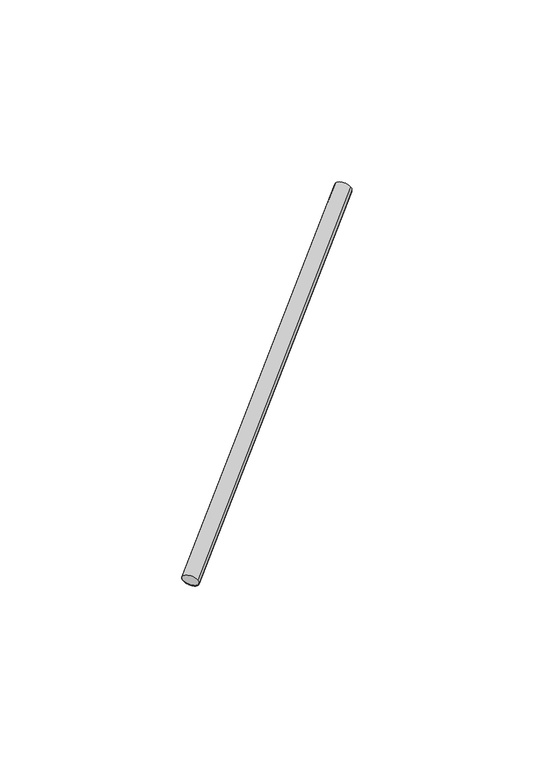
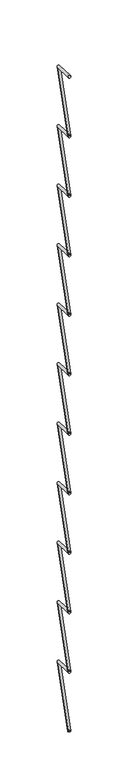
"""IFC4 building model written with IfcOpenShell, lengths in millimetres: proxy geometry, Vigota 7 (Pano 3) (Mf = 137)."""

from ifc_helpers import new_model, si_unit, point, frame, origin, origin_2d, place, context, project, spatial, circle_curve, trimmed, segment, composite_curve, outline, extrude, source, transform, mapped, element, save


def structural_framing_98597a9d(model_context):
    return source(origin(), model_context, "Body", "SweptSolid", [
        extrude(outline(composite_curve([segment(trimmed(circle_curve(origin_2d(), 2.5), [point((2.5, 0.0))], [point((-2.5, 0.0))], False, "CARTESIAN"), True, "CONTINUOUS"), segment(trimmed(circle_curve(origin_2d(), 2.5), [point((-2.5, 0.0))], [point((2.5, 0.0))], False, "CARTESIAN"), True, "CONTINUOUS")], self_intersect=False)), frame((-42.0, 0.0, 1737.500535), z_axis=(0.3218603428886276, 0.8276408817707567, 0.4598004898837537), x_axis=(0.8192319205108605, 3.936835275445103e-11, -0.5734623443750141)), (0.0, 0.0, 1.0), 130.491379),
        extrude(outline(composite_curve([segment(trimmed(circle_curve(origin_2d(), 2.5), [point((2.5, 0.0))], [point((-2.5, 0.0))], False, "CARTESIAN"), True, "CONTINUOUS"), segment(trimmed(circle_curve(origin_2d(), 2.5), [point((-2.5, 0.0))], [point((2.5, 0.0))], False, "CARTESIAN"), True, "CONTINUOUS")], self_intersect=False)), frame((0.0, 108.0, 1797.500535), z_axis=(-0.3218603428886276, -0.8276408817707567, 0.4598004898837537), x_axis=(0.8192319205108605, 3.936835275445103e-11, 0.5734623443750141)), (0.0, 0.0, 1.0), 130.491379),
        extrude(outline(composite_curve([segment(trimmed(circle_curve(origin_2d(), 2.5), [point((2.5, 0.0))], [point((-2.5, 0.0))], False, "CARTESIAN"), True, "CONTINUOUS"), segment(trimmed(circle_curve(origin_2d(), 2.5), [point((-2.5, 0.0))], [point((2.5, 0.0))], False, "CARTESIAN"), True, "CONTINUOUS")], self_intersect=False)), frame((-42.0, 0.0, 1857.500535), z_axis=(0.3218603428886276, 0.8276408817707567, 0.4598004898837537), x_axis=(0.8192319205108605, 3.936835275445103e-11, -0.5734623443750141)), (0.0, 0.0, 1.0), 130.491379),
        extrude(outline(composite_curve([segment(trimmed(circle_curve(origin_2d(), 2.5), [point((2.5, 0.0))], [point((-2.5, 0.0))], False, "CARTESIAN"), True, "CONTINUOUS"), segment(trimmed(circle_curve(origin_2d(), 2.5), [point((-2.5, 0.0))], [point((2.5, 0.0))], False, "CARTESIAN"), True, "CONTINUOUS")], self_intersect=False)), frame((0.0, 108.0, 1917.500535), z_axis=(-0.3218603428886276, -0.8276408817707567, 0.4598004898837537), x_axis=(0.8192319205108605, 3.936835275445103e-11, 0.5734623443750141)), (0.0, 0.0, 1.0), 130.491379),
        extrude(outline(composite_curve([segment(trimmed(circle_curve(origin_2d(), 2.5), [point((2.5, 0.0))], [point((-2.5, 0.0))], False, "CARTESIAN"), True, "CONTINUOUS"), segment(trimmed(circle_curve(origin_2d(), 2.5), [point((-2.5, 0.0))], [point((2.5, 0.0))], False, "CARTESIAN"), True, "CONTINUOUS")], self_intersect=False)), frame((-42.0, 0.0, 1977.500535), z_axis=(0.3218603428886276, 0.8276408817707567, 0.4598004898837537), x_axis=(0.8192319205108605, 3.936835275445103e-11, -0.5734623443750141)), (0.0, 0.0, 1.0), 130.491379),
        extrude(outline(composite_curve([segment(trimmed(circle_curve(origin_2d(), 2.5), [point((2.5, 0.0))], [point((-2.5, 0.0))], False, "CARTESIAN"), True, "CONTINUOUS"), segment(trimmed(circle_curve(origin_2d(), 2.5), [point((-2.5, 0.0))], [point((2.5, 0.0))], False, "CARTESIAN"), True, "CONTINUOUS")], self_intersect=False)), frame((0.0, 108.0, 2037.500535), z_axis=(-0.3218603428886276, -0.8276408817707567, 0.4598004898837537), x_axis=(0.8192319205108605, 3.936835275445103e-11, 0.5734623443750141)), (0.0, 0.0, 1.0), 130.491379),
        extrude(outline(composite_curve([segment(trimmed(circle_curve(origin_2d(), 2.5), [point((2.5, 0.0))], [point((-2.5, 0.0))], False, "CARTESIAN"), True, "CONTINUOUS"), segment(trimmed(circle_curve(origin_2d(), 2.5), [point((-2.5, 0.0))], [point((2.5, 0.0))], False, "CARTESIAN"), True, "CONTINUOUS")], self_intersect=False)), frame((-42.0, 0.0, 2097.500535), z_axis=(0.3218603428886276, 0.8276408817707567, 0.4598004898837537), x_axis=(0.8192319205108605, 3.936835275445103e-11, -0.5734623443750141)), (0.0, 0.0, 1.0), 130.491379),
        extrude(outline(composite_curve([segment(trimmed(circle_curve(origin_2d(), 2.5), [point((2.5, 0.0))], [point((-2.5, 0.0))], False, "CARTESIAN"), True, "CONTINUOUS"), segment(trimmed(circle_curve(origin_2d(), 2.5), [point((-2.5, 0.0))], [point((2.5, 0.0))], False, "CARTESIAN"), True, "CONTINUOUS")], self_intersect=False)), frame((0.0, 108.0, 2157.500535), z_axis=(-0.3218603428886276, -0.8276408817707567, 0.4598004898837537), x_axis=(0.8192319205108605, 3.936835275445103e-11, 0.5734623443750141)), (0.0, 0.0, 1.0), 130.491379),
        extrude(outline(composite_curve([segment(trimmed(circle_curve(origin_2d(), 2.5), [point((2.5, 0.0))], [point((-2.5, 0.0))], False, "CARTESIAN"), True, "CONTINUOUS"), segment(trimmed(circle_curve(origin_2d(), 2.5), [point((-2.5, 0.0))], [point((2.5, 0.0))], False, "CARTESIAN"), True, "CONTINUOUS")], self_intersect=False)), frame((-42.0, 0.0, 2217.500535), z_axis=(0.3218603428886276, 0.8276408817707567, 0.4598004898837537), x_axis=(0.8192319205108605, 3.936835275445103e-11, -0.5734623443750141)), (0.0, 0.0, 1.0), 130.491379),
        extrude(outline(composite_curve([segment(trimmed(circle_curve(origin_2d(), 2.5), [point((2.5, 0.0))], [point((-2.5, 0.0))], False, "CARTESIAN"), True, "CONTINUOUS"), segment(trimmed(circle_curve(origin_2d(), 2.5), [point((-2.5, 0.0))], [point((2.5, 0.0))], False, "CARTESIAN"), True, "CONTINUOUS")], self_intersect=False)), frame((0.0, 108.0, 2277.500535), z_axis=(-0.3218603428886276, -0.8276408817707567, 0.4598004898837537), x_axis=(0.8192319205108605, 3.936835275445103e-11, 0.5734623443750141)), (0.0, 0.0, 1.0), 130.491379),
        extrude(outline(composite_curve([segment(trimmed(circle_curve(origin_2d(), 2.5), [point((2.5, 0.0))], [point((-2.5, 0.0))], False, "CARTESIAN"), True, "CONTINUOUS"), segment(trimmed(circle_curve(origin_2d(), 2.5), [point((-2.5, 0.0))], [point((2.5, 0.0))], False, "CARTESIAN"), True, "CONTINUOUS")], self_intersect=False)), frame((-42.0, 0.0, 2337.500535), z_axis=(0.3218603428886276, 0.8276408817707567, 0.4598004898837537), x_axis=(0.8192319205108605, 3.936835275445103e-11, -0.5734623443750141)), (0.0, 0.0, 1.0), 130.491379),
        extrude(outline(composite_curve([segment(trimmed(circle_curve(origin_2d(), 2.5), [point((2.5, 0.0))], [point((-2.5, 0.0))], False, "CARTESIAN"), True, "CONTINUOUS"), segment(trimmed(circle_curve(origin_2d(), 2.5), [point((-2.5, 0.0))], [point((2.5, 0.0))], False, "CARTESIAN"), True, "CONTINUOUS")], self_intersect=False)), frame((0.0, 108.0, 2397.500535), z_axis=(-0.3218603428886276, -0.8276408817707567, 0.4598004898837537), x_axis=(0.8192319205108605, 3.936835275445103e-11, 0.5734623443750141)), (0.0, 0.0, 1.0), 130.491379),
        extrude(outline(composite_curve([segment(trimmed(circle_curve(origin_2d(), 2.5), [point((2.5, 0.0))], [point((-2.5, 0.0))], False, "CARTESIAN"), True, "CONTINUOUS"), segment(trimmed(circle_curve(origin_2d(), 2.5), [point((-2.5, 0.0))], [point((2.5, 0.0))], False, "CARTESIAN"), True, "CONTINUOUS")], self_intersect=False)), frame((-42.0, 0.0, 2457.500535), z_axis=(0.3218603428886276, 0.8276408817707567, 0.4598004898837537), x_axis=(0.8192319205108605, 3.936835275445103e-11, -0.5734623443750141)), (0.0, 0.0, 1.0), 130.491379),
        extrude(outline(composite_curve([segment(trimmed(circle_curve(origin_2d(), 2.5), [point((2.5, 0.0))], [point((-2.5, 0.0))], False, "CARTESIAN"), True, "CONTINUOUS"), segment(trimmed(circle_curve(origin_2d(), 2.5), [point((-2.5, 0.0))], [point((2.5, 0.0))], False, "CARTESIAN"), True, "CONTINUOUS")], self_intersect=False)), frame((0.0, 108.0, 2517.500535), z_axis=(-0.3218603428886276, -0.8276408817707567, 0.4598004898837537), x_axis=(0.8192319205108605, 3.936835275445103e-11, 0.5734623443750141)), (0.0, 0.0, 1.0), 130.491379),
        extrude(outline(composite_curve([segment(trimmed(circle_curve(origin_2d(), 2.5), [point((2.5, 0.0))], [point((-2.5, 0.0))], False, "CARTESIAN"), True, "CONTINUOUS"), segment(trimmed(circle_curve(origin_2d(), 2.5), [point((-2.5, 0.0))], [point((2.5, 0.0))], False, "CARTESIAN"), True, "CONTINUOUS")], self_intersect=False)), frame((-42.0, 0.0, 2577.500535), z_axis=(0.3218603428886276, 0.8276408817707567, 0.4598004898837537), x_axis=(0.8192319205108605, 3.936835275445103e-11, -0.5734623443750141)), (0.0, 0.0, 1.0), 130.491379),
        extrude(outline(composite_curve([segment(trimmed(circle_curve(origin_2d(), 2.5), [point((2.5, 0.0))], [point((-2.5, 0.0))], False, "CARTESIAN"), True, "CONTINUOUS"), segment(trimmed(circle_curve(origin_2d(), 2.5), [point((-2.5, 0.0))], [point((2.5, 0.0))], False, "CARTESIAN"), True, "CONTINUOUS")], self_intersect=False)), frame((0.0, 108.0, 2637.500535), z_axis=(-0.3218603428886276, -0.8276408817707567, 0.4598004898837537), x_axis=(0.8192319205108605, 3.936835275445103e-11, 0.5734623443750141)), (0.0, 0.0, 1.0), 130.491379),
        extrude(outline(composite_curve([segment(trimmed(circle_curve(origin_2d(), 2.5), [point((2.5, 0.0))], [point((-2.5, 0.0))], False, "CARTESIAN"), True, "CONTINUOUS"), segment(trimmed(circle_curve(origin_2d(), 2.5), [point((-2.5, 0.0))], [point((2.5, 0.0))], False, "CARTESIAN"), True, "CONTINUOUS")], self_intersect=False)), frame((-42.0, 0.0, 2697.500535), z_axis=(0.3218603428886276, 0.8276408817707567, 0.4598004898837537), x_axis=(0.8192319205108605, 3.936835275445103e-11, -0.5734623443750141)), (0.0, 0.0, 1.0), 130.491379),
        extrude(outline(composite_curve([segment(trimmed(circle_curve(origin_2d(), 2.5), [point((2.5, 0.0))], [point((-2.5, 0.0))], False, "CARTESIAN"), True, "CONTINUOUS"), segment(trimmed(circle_curve(origin_2d(), 2.5), [point((-2.5, 0.0))], [point((2.5, 0.0))], False, "CARTESIAN"), True, "CONTINUOUS")], self_intersect=False)), frame((0.0, 108.0, 2757.500535), z_axis=(-0.3218603428886276, -0.8276408817707567, 0.4598004898837537), x_axis=(0.8192319205108605, 3.936835275445103e-11, 0.5734623443750141)), (0.0, 0.0, 1.0), 130.491379),
        extrude(outline(composite_curve([segment(trimmed(circle_curve(origin_2d(), 2.5), [point((2.5, 0.0))], [point((-2.5, 0.0))], False, "CARTESIAN"), True, "CONTINUOUS"), segment(trimmed(circle_curve(origin_2d(), 2.5), [point((-2.5, 0.0))], [point((2.5, 0.0))], False, "CARTESIAN"), True, "CONTINUOUS")], self_intersect=False)), frame((-42.0, 0.0, 2817.500535), z_axis=(0.3218603428886276, 0.8276408817707567, 0.4598004898837537), x_axis=(0.8192319205108605, 3.936835275445103e-11, -0.5734623443750141)), (0.0, 0.0, 1.0), 130.491379),
        extrude(outline(composite_curve([segment(trimmed(circle_curve(origin_2d(), 2.5), [point((2.5, 0.0))], [point((-2.5, 0.0))], False, "CARTESIAN"), True, "CONTINUOUS"), segment(trimmed(circle_curve(origin_2d(), 2.5), [point((-2.5, 0.0))], [point((2.5, 0.0))], False, "CARTESIAN"), True, "CONTINUOUS")], self_intersect=False)), frame((0.0, 108.0, 2877.500535), z_axis=(-0.3218603428886276, -0.8276408817707567, 0.4598004898837537), x_axis=(0.8192319205108605, 3.936835275445103e-11, 0.5734623443750141)), (0.0, 0.0, 1.0), 130.491379),
        extrude(outline(composite_curve([segment(trimmed(circle_curve(origin_2d(), 2.5), [point((2.5, 0.0))], [point((-2.5, 0.0))], False, "CARTESIAN"), True, "CONTINUOUS"), segment(trimmed(circle_curve(origin_2d(), 2.5), [point((-2.5, 0.0))], [point((2.5, 0.0))], False, "CARTESIAN"), True, "CONTINUOUS")], self_intersect=False)), frame((-42.0, 0.0, 2937.500535), z_axis=(0.3218603428886276, 0.8276408817707567, 0.4598004898837537), x_axis=(0.8192319205108605, 3.936835275445103e-11, -0.5734623443750141)), (0.0, 0.0, 1.0), 130.491379),
        extrude(outline(composite_curve([segment(trimmed(circle_curve(origin_2d(), 2.5), [point((2.5, 0.0))], [point((-2.5, 0.0))], False, "CARTESIAN"), True, "CONTINUOUS"), segment(trimmed(circle_curve(origin_2d(), 2.5), [point((-2.5, 0.0))], [point((2.5, 0.0))], False, "CARTESIAN"), True, "CONTINUOUS")], self_intersect=False)), frame((0.0, 108.0, 2997.500535), z_axis=(-0.3218603428886276, -0.8276408817707567, 0.4598004898837537), x_axis=(0.8192319205108605, 3.936835275445103e-11, 0.5734623443750141)), (0.0, 0.0, 1.0), 130.491379),
    ])


if __name__ == "__main__":
    model = new_model("IFC4")
    model_context = context("Model", 3, world=origin())
    ifc_project = project(units=[si_unit("LENGTHUNIT", "METRE", prefix="MILLI")], contexts=[model_context])
    site = spatial("IfcSite", under=ifc_project)
    building = spatial("IfcBuilding", under=site)
    placement = place(None, origin())
    structural_framing_shape = structural_framing_98597a9d(model_context)
    element("IfcBuildingElementProxy", 1, Name="Vigota 7 (Pano 3) (Mf = 137)", ObjectType="Vigota 7 (Pano 3) (Mf = 137)", at=placement, inside=building, context=model_context, shape_type="MappedRepresentation", body=[
        mapped(structural_framing_shape, transform((0.0, 0.0, 0.0), x_axis=(1.0, 0.0, 0.0), y_axis=(0.0, 1.0, 0.0), z_axis=(0.0, 0.0, 1.0))),
    ])
    save(model, "model.ifc")

# Revit data of these elements
# Element 1 (IfcBuildingElementProxy, "Vigota 7 (Pano 3) (Mf = 137)")
#   Materials on its faces: "Aço", "Concreto armado"
# Materials
#   "Aço": class "Metal", colour RGB 120 120 120, transparency 0, Description = "Aço estrutural A36 grau, ASTM B, acabamento laminado", Cost = 0
#   "Concreto armado": class "Não atribuído", colour RGB 168 169 158, transparency 0
